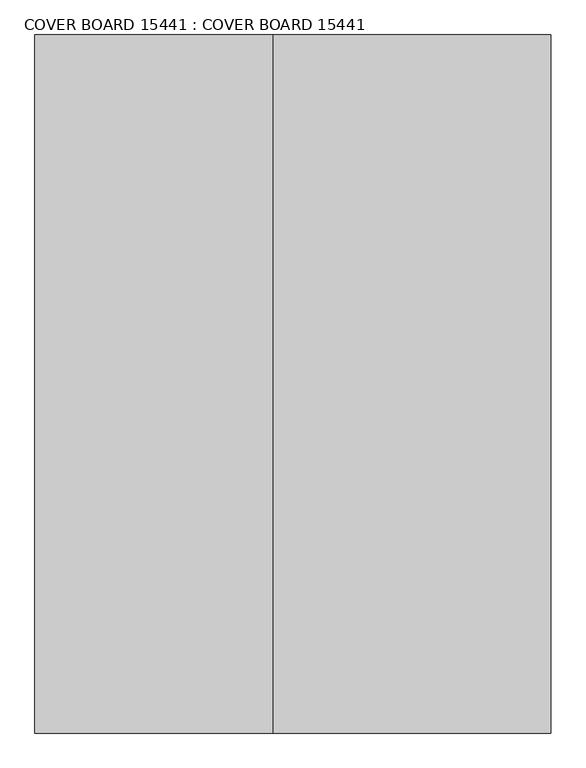
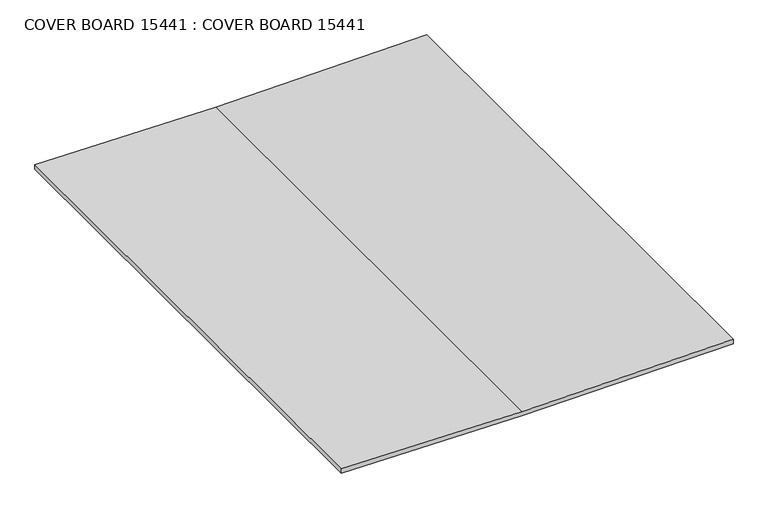
"""IFC4 building model written with IfcOpenShell, lengths in millimetres: proxy geometry, COVER BOARD 15441 : COVER BOARD 15441."""

import ifcopenshell
import ifcopenshell.guid

model = None  # the IFC model being written
_history = None  # IfcOwnerHistory: only IFC2X3 demands one
_inside = {}  # id of a spatial element -> (the spatial element, [elements in it])
_under = {}  # id of a project, library or spatial element -> (it, [spatial elements below it])
_declared = {}  # id of a project -> (the project, [libraries it declares])
_typed = {}  # id of a type object -> (the type object, [elements of that type])
_made_of = {}  # id of a material, layer set ... -> (it, [elements and type objects made of it])


def new_model(schema):
    """Start an empty IFC model of exactly this schema.

    Asked for "IFC4X3", IfcOpenShell would pick the latest addendum, in which some entities
    have other attributes; the version numbers below select the first issue.
    IFC2X3 requires an IfcOwnerHistory on every rooted entity: one is made here for all.
    """
    global model, _history
    if schema == "IFC4X3":
        model = ifcopenshell.file(schema_version=(4, 3, 0, 0))
    else:
        model = ifcopenshell.file(schema=schema)
    _inside.clear()
    _under.clear()
    _declared.clear()
    _typed.clear()
    _made_of.clear()
    _history = None
    if model.schema == "IFC2X3":
        org = make("IfcOrganization", Name="unknown")
        user = make(
            "IfcPersonAndOrganization",
            ThePerson=make("IfcPerson", FamilyName="unknown"),
            TheOrganization=org,
        )
        app = make(
            "IfcApplication",
            ApplicationDeveloper=org,
            Version="unknown",
            ApplicationFullName="unknown",
            ApplicationIdentifier="unknown",
        )
        _history = make(
            "IfcOwnerHistory",
            OwningUser=user,
            OwningApplication=app,
            ChangeAction="ADDED",
            CreationDate=0,
        )
    return model


def make(cls, **values):
    """One entity of the class cls with the attributes given. An attribute that is None is left unset."""
    return model.create_entity(
        cls, **{name: value for name, value in values.items() if value is not None}
    )


def rooted(cls, **values):
    """An entity with a GlobalId (a new one), such as an element, a storey or a relation."""
    return make(cls, GlobalId=ifcopenshell.guid.new(), OwnerHistory=_history, **values)


def si_unit(unit_type, name, prefix=None):
    """IfcSIUnit, for example si_unit("LENGTHUNIT", "METRE", prefix="MILLI")."""
    return make("IfcSIUnit", UnitType=unit_type, Prefix=prefix, Name=name)


def assignment(units):
    """IfcUnitAssignment: the units of a project."""
    return None if units is None else make("IfcUnitAssignment", Units=units)


def point(xyz):
    """IfcCartesianPoint."""
    return None if xyz is None else make("IfcCartesianPoint", Coordinates=xyz)


def direction(xyz):
    """IfcDirection."""
    return None if xyz is None else make("IfcDirection", DirectionRatios=xyz)


def frame(location, z_axis=None, x_axis=None):
    """IfcAxis2Placement3D, a coordinate frame: its origin and axes. An axis left out is left unset."""
    return make(
        "IfcAxis2Placement3D",
        Location=point(location),
        Axis=direction(z_axis),
        RefDirection=direction(x_axis),
    )


def origin():
    """The frame at (0, 0, 0) with its axes left unset."""
    return frame((0.0, 0.0, 0.0))


def place(relative_to, where):
    """IfcLocalPlacement: puts the frame where relative to a parent placement (None: the world)."""
    return make(
        "IfcLocalPlacement", PlacementRelTo=relative_to, RelativePlacement=where
    )


def context(
    kind, dimensions, precision=None, world=None, true_north=None, identifier=None
):
    """IfcGeometricRepresentationContext, for example the 3D "Model" context."""
    return make(
        "IfcGeometricRepresentationContext",
        ContextIdentifier=identifier,
        ContextType=kind,
        CoordinateSpaceDimension=dimensions,
        Precision=precision,
        WorldCoordinateSystem=world,
        TrueNorth=true_north,
    )


def project(units=None, contexts=None):
    """IfcProject with its units and contexts."""
    return rooted(
        "IfcProject",
        Name="project",
        RepresentationContexts=contexts,
        UnitsInContext=assignment(units),
    )


def spatial(cls, under=None, at=None, **own):
    """A site, building, storey or space (cls), placed at a placement, below another one or the project."""
    s = rooted(cls, ObjectPlacement=at, **own)
    if under is not None:
        _under.setdefault(under.id(), (under, []))[1].append(s)
    return s


def polyline(points):
    """IfcPolyline through the points."""
    return make("IfcPolyline", Points=[point(p) for p in points])


def outline(outer, holes=None, kind="AREA"):
    """IfcArbitraryClosedProfileDef: a profile drawn as a closed curve; with holes, ...WithVoids."""
    if holes is None:
        return make("IfcArbitraryClosedProfileDef", ProfileType=kind, OuterCurve=outer)
    return make(
        "IfcArbitraryProfileDefWithVoids",
        ProfileType=kind,
        OuterCurve=outer,
        InnerCurves=holes,
    )


def extrude(swept, where, along, depth):
    """IfcExtrudedAreaSolid: the profile swept, set in the frame where, extruded along a direction by depth."""
    return make(
        "IfcExtrudedAreaSolid",
        SweptArea=swept,
        Position=where,
        ExtrudedDirection=direction(along),
        Depth=depth,
    )


def shape(context_of_items, identifier, shape_type, items):
    """IfcShapeRepresentation: the items that make up one representation, for example the "Body"."""
    return make(
        "IfcShapeRepresentation",
        ContextOfItems=context_of_items,
        RepresentationIdentifier=identifier,
        RepresentationType=shape_type,
        Items=items,
    )


def source(mapping_origin, context_of_items, identifier, shape_type, items):
    """IfcRepresentationMap: a shape defined once, which mapped items show again and again."""
    return make(
        "IfcRepresentationMap",
        MappingOrigin=mapping_origin,
        MappedRepresentation=shape(context_of_items, identifier, shape_type, items),
    )


def transform(
    local_origin,
    x_axis=None,
    y_axis=None,
    z_axis=None,
    scale=None,
    scale2=None,
    scale3=None,
    uniform=True,
):
    """IfcCartesianTransformationOperator3D, or its non-uniform kind. x_axis, y_axis, z_axis: its Axis1, 2, 3."""
    if uniform:
        return make(
            "IfcCartesianTransformationOperator3D",
            Axis1=direction(x_axis),
            Axis2=direction(y_axis),
            LocalOrigin=point(local_origin),
            Scale=scale,
            Axis3=direction(z_axis),
        )
    return make(
        "IfcCartesianTransformationOperator3DnonUniform",
        Axis1=direction(x_axis),
        Axis2=direction(y_axis),
        LocalOrigin=point(local_origin),
        Scale=scale,
        Axis3=direction(z_axis),
        Scale2=scale2,
        Scale3=scale3,
    )


def mapped(mapping_source, mapping_target):
    """IfcMappedItem: shows the shape of a source again, moved by a transform."""
    return make(
        "IfcMappedItem", MappingSource=mapping_source, MappingTarget=mapping_target
    )


def made_of(thing, what):
    """Note that an element or type object is made of a material, layer set ...; save() writes the relation."""
    if what is not None:
        _made_of.setdefault(what.id(), (what, []))[1].append(thing)
    return thing


def element(
    cls,
    number,
    at=None,
    inside=None,
    cuts=None,
    type_object=None,
    material=None,
    context=None,
    identifier="Body",
    shape_type=None,
    held_by="IfcProductDefinitionShape",
    body=None,
    shapes=None,
    **own,
):
    """One element of the class cls, such as IfcWall. Its Tag is "e" and its number.

    at: its placement. inside: the storey or other place that contains it. cuts: it is an
    opening in that element (IfcRelVoidsElement). A single representation is given by context,
    identifier, shape_type and body (its items); several are given by shapes. held_by: the class
    of the entity that holds the representations. save() writes the other relations.
    """
    e = rooted(cls, Tag="e%d" % number, ObjectPlacement=at, **own)
    if body is not None:
        shapes = [shape(context, identifier, shape_type, body)]
    if shapes is not None:
        e.Representation = make(held_by, Representations=shapes)
    if inside is not None:
        _inside.setdefault(inside.id(), (inside, []))[1].append(e)
    if cuts is not None:
        rooted(
            "IfcRelVoidsElement", RelatingBuildingElement=cuts, RelatedOpeningElement=e
        )
    if type_object is not None:
        _typed.setdefault(type_object.id(), (type_object, []))[1].append(e)
    return made_of(e, material)


def aggregate(whole, parts):
    """IfcRelAggregates: a whole, such as a stair, and the parts it consists of."""
    return rooted("IfcRelAggregates", RelatingObject=whole, RelatedObjects=parts)


def save(model, path):
    """Write the relations noted so far, then the file.

    IfcRelAggregates (storeys below a building ...), IfcRelContainedInSpatialStructure (elements
    in a storey), IfcRelDefinesByType, IfcRelAssociatesMaterial and IfcRelDeclares: one each for
    every whole, place, type object, material and project.
    """
    for whole, parts in _under.values():
        aggregate(whole, parts)
    for where, things in _inside.values():
        rooted(
            "IfcRelContainedInSpatialStructure",
            RelatedElements=things,
            RelatingStructure=where,
        )
    for kind, things in _typed.values():
        rooted("IfcRelDefinesByType", RelatedObjects=things, RelatingType=kind)
    for what, things in _made_of.values():
        rooted("IfcRelAssociatesMaterial", RelatedObjects=things, RelatingMaterial=what)
    for by, libraries in _declared.values():
        rooted("IfcRelDeclares", RelatingContext=by, RelatedDefinitions=libraries)
    model.write(path)


def cover_board_15441_cover_board_15441_a2131a35(model_context):
    return source(origin(), model_context, "Body", "SweptSolid", [
        extrude(outline(polyline([(40228.1021556, -1886.5629484), (40237.9000089, -2567.3737014), (40220.5682898, -2567.3737014), (40210.7704365, -1886.5629484), (40220.5682898, -1090.0815411), (40237.9000089, -1090.0815411), (40228.1021556, -1886.5629484)])), frame((0.0, -1052.6406573, 0.0), z_axis=(0.0, 1.0, 0.0), x_axis=(0.0, 0.0, 1.0)), (0.0, 0.0, 1.0), 2000.0),
    ])


if __name__ == "__main__":
    model = new_model("IFC4")
    model_context = context("Model", 3, world=origin())
    ifc_project = project(units=[si_unit("LENGTHUNIT", "METRE", prefix="MILLI")], contexts=[model_context])
    site = spatial("IfcSite", under=ifc_project)
    building = spatial("IfcBuilding", under=site)
    placement = place(None, origin())
    cover_board_15441_cover_board_15441_shape = cover_board_15441_cover_board_15441_a2131a35(model_context)
    element("IfcBuildingElementProxy", 1, Name="COVER BOARD 15441 : COVER BOARD 15441", ObjectType="COVER BOARD 15441 : COVER BOARD 15441", at=placement, inside=building, context=model_context, shape_type="MappedRepresentation", body=[
        mapped(cover_board_15441_cover_board_15441_shape, transform((0.0, 0.0, 0.0), x_axis=(1.0, 0.0, 0.0), y_axis=(0.0, 1.0, 0.0), z_axis=(0.0, 0.0, 1.0))),
    ])
    save(model, "model.ifc")

# Revit data of these elements
# Type "COVER BOARD 15441 : COVER BOARD 15441"
#   NameOverride = "COVER BOARD"
# Element 1 (IfcBuildingElementProxy, "COVER BOARD 15441 : COVER BOARD 15441")
#   Materials on its faces: "CDX PLYWOOD - SEE STRUCTURAL DWGS"
# Materials
#   "CDX PLYWOOD - SEE STRUCTURAL DWGS": class "Unassigned", colour RGB 202 163 108, transparency 0, Cost = 0
